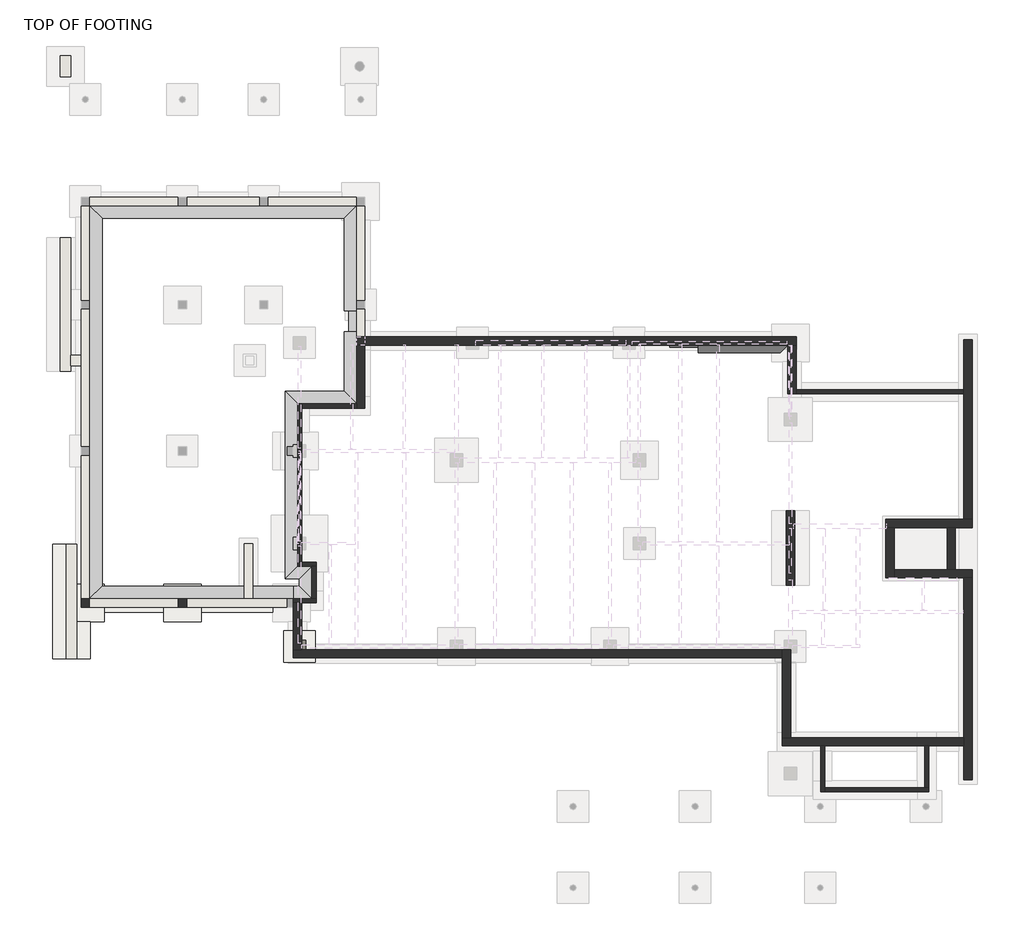
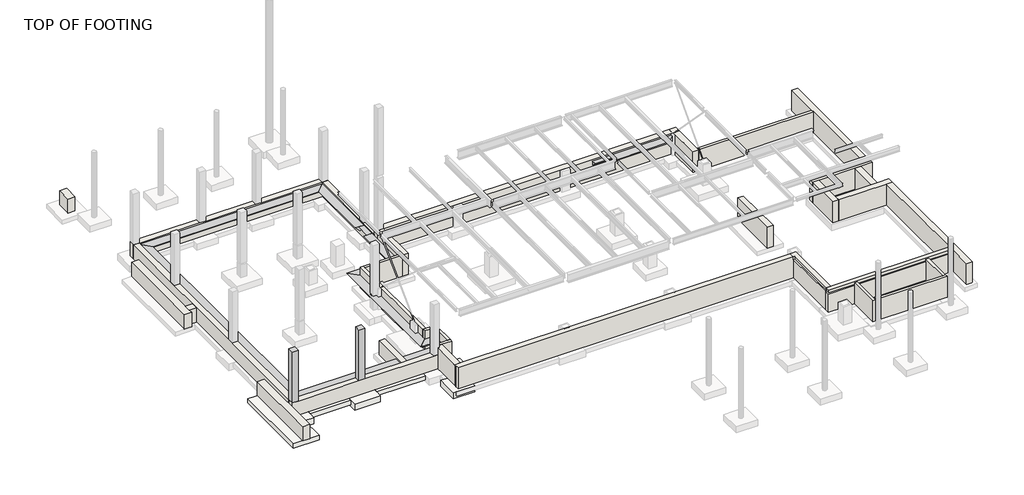
# One storey, part 1 of 4: 32 walls, 8 proxies, 3 slabs, 2 columns, 2 footings.
# Revit data of these elements (continued)
# Element 20 (IfcWall, "Foundation - 16\" Concrete") (continued)
#   RM User Number = 221
#   RM Unique Id = 1041
#   RS Unique Id = 299748
#   Phase Created = New Construction
#   Base Constraint = TOP OF FOOTING
#   Top Constraint = Ground Floor
#   Materials on its faces: "Concrete, Normal Weight - 4 ksi"
# Element 21 (IfcWall, "Foundation - 16\" Concrete")
#   Comments = ""
#   Top Offset = 0 mm
#   Base Offset = 0 mm
#   wall height = 1574.8 mm
#   RM User Number = 222
#   RM Unique Id = 1042
#   RS Unique Id = 299919
#   Phase Created = New Construction
#   Base Constraint = TOP OF FOOTING
#   Top Constraint = Ground Floor
#   Materials on its faces: "Concrete, Normal Weight - 4 ksi"
# Element 22 (IfcWall, "Foundation - 16\" Concrete")
#   Comments = ""
#   Top Offset = 0 mm
#   Base Offset = 0 mm
#   wall height = 1066.8 mm
#   RM User Number = 223
#   RM Unique Id = 1043
#   RS Unique Id = 300105
#   Phase Created = New Construction
#   Base Constraint = TOP OF FOOTING
#   Top Constraint = LOWER LEVEL
#   Materials on its faces: "Concrete, Normal Weight - 4 ksi"
# Element 23 (IfcWall, "Foundation - 16\" Concrete")
#   Comments = ""
#   Top Offset = 0 mm
#   Base Offset = 0 mm
#   wall height = 1066.8 mm
#   RM User Number = 224
#   RM Unique Id = 1044
#   RS Unique Id = 300160
#   Phase Created = New Construction
#   Base Constraint = TOP OF FOOTING
#   Top Constraint = LOWER LEVEL
#   Materials on its faces: "Concrete, Normal Weight - 4 ksi"
# Element 24 (IfcWall, "Foundation - 16\" Concrete")
#   Comments = ""
#   Top Offset = 0 mm
#   Base Offset = 0 mm
#   wall height = 1066.8 mm
#   RM User Number = 225
#   RM Unique Id = 1045
#   RS Unique Id = 300261
#   Phase Created = New Construction
#   Base Constraint = TOP OF FOOTING
#   Top Constraint = LOWER LEVEL
#   Materials on its faces: "Concrete, Normal Weight - 4 ksi"
# Element 25 (IfcWall, "Foundation - 16\" Concrete")
#   Comments = ""
#   Top Offset = 0 mm
#   Base Offset = 0 mm
#   wall height = 1066.8 mm
#   RM User Number = 226
#   RM Unique Id = 1046
#   RS Unique Id = 300335
#   Phase Created = New Construction
#   Base Constraint = TOP OF FOOTING
#   Top Constraint = LOWER LEVEL
#   Materials on its faces: "Concrete, Normal Weight - 4 ksi"
# Element 26 (IfcWall, "Foundation - 16\" Concrete")
#   Comments = ""
#   Top Offset = 0 mm
#   Base Offset = 0 mm
#   wall height = 1574.8 mm
#   RM User Number = 228
#   RM Unique Id = 1048
#   RS Unique Id = 300755
#   Phase Created = New Construction
#   Base Constraint = TOP OF FOOTING
#   Top Constraint = Ground Floor
#   Materials on its faces: "Concrete, Normal Weight - 4 ksi", "Concrete, Cast-in-Place gray"
# Element 27 (IfcWall, "Foundation - 16\" Concrete")
#   Comments = ""
#   Top Offset = 0 mm
#   Base Offset = 0 mm
#   wall height = 1574.8 mm
#   RM User Number = 231
#   RM Unique Id = 1055
#   RS Unique Id = 301226
#   Phase Created = New Construction
#   Base Constraint = TOP OF FOOTING
#   Top Constraint = Ground Floor
#   Materials on its faces: "Concrete, Normal Weight - 4 ksi"
# Element 28 (IfcWall, "Foundation - 16\" Concrete")
#   Comments = ""
#   Top Offset = 0 mm
#   Base Offset = 0 mm
#   wall height = 1574.8 mm
#   RM User Number = 232
#   RM Unique Id = 1056
#   RS Unique Id = 301303
#   Phase Created = New Construction
#   Base Constraint = TOP OF FOOTING
#   Top Constraint = Ground Floor
#   Materials on its faces: "Concrete, Normal Weight - 4 ksi"
# Element 29 (IfcWall, "Foundation - 16\" Concrete")
#   Comments = ""
#   Top Offset = 0 mm
#   Base Offset = 0 mm
#   wall height = 1574.8 mm
#   RM User Number = 233
#   RM Unique Id = 1057
#   RS Unique Id = 301434
#   Phase Created = New Construction
#   Base Constraint = TOP OF FOOTING
#   Top Constraint = Ground Floor
#   Materials on its faces: "Concrete, Normal Weight - 4 ksi"
# Element 30 (IfcWall, "Foundation - 16\" Concrete")
#   Comments = ""
#   Top Offset = 0 mm
#   Base Offset = 0 mm
#   wall height = 1066.8 mm
#   RM User Number = 252
#   RM Unique Id = 1092
#   RS Unique Id = 386049
#   Phase Created = New Construction
#   Base Constraint = TOP OF FOOTING
#   Top Constraint = LOWER LEVEL
#   Materials on its faces: "Concrete, Normal Weight - 4 ksi"
# Element 31 (IfcWall, "Foundation - 16\" Concrete")
#   Top Offset = 0 mm
#   Base Offset = 0 mm
#   wall height = 1574.8 mm
#   RM User Number = 253
#   RM Unique Id = 1093
#   RS Unique Id = 386870
#   Phase Created = New Construction
#   Base Constraint = TOP OF FOOTING
#   Top Constraint = Ground Floor
#   Materials on its faces: "Concrete, Normal Weight - 4 ksi"
# Element 32 (IfcWall, "Foundation - 16\" Concrete")
#   Comments = ""
#   Top Offset = 0 mm
#   Base Offset = 0 mm
#   wall height = 1574.8 mm
#   RM User Number = 261
#   RM Unique Id = 1108
#   RS Unique Id = 398252
#   Phase Created = New Construction
#   Base Constraint = TOP OF FOOTING
#   Top Constraint = Ground Floor
#   Materials on its faces: "Concrete, Normal Weight - 4 ksi"
# Element 33 (IfcWall, "Foundation - 16\" Concrete w/Brick Ledge")
#   Comments = ""
#   Top Offset = 0 mm
#   Base Offset = 0 mm
#   wall height = 1574.8 mm
#   RM User Number = 218
#   RM Unique Id = 1036
#   RS Unique Id = 299490
#   Phase Created = New Construction
#   Base Constraint = TOP OF FOOTING
#   Top Constraint = Ground Floor
#   Materials on its faces: "Concrete, Cast-in-Place gray"
# Element 34 (IfcWall, "Foundation - 16\" Concrete w/Brick Ledge")
#   Comments = ""
#   Top Offset = 0 mm
#   Base Offset = 0 mm
#   wall height = 1574.8 mm
#   RM User Number = 219
#   RM Unique Id = 1039
#   RS Unique Id = 299551
#   Phase Created = New Construction
#   Base Constraint = TOP OF FOOTING
#   Top Constraint = Ground Floor
#   Materials on its faces: "Concrete, Cast-in-Place gray", "Concrete, Normal Weight - 4 ksi"
# Element 35 (IfcWall, "Foundation - 20\" Concrete")
#   Comments = ""
#   Top Offset = 0 mm
#   Base Offset = 0 mm
#   wall height = 1066.8 mm
#   RM User Number = 249
#   RM Unique Id = 1087
#   RS Unique Id = 384622
#   Phase Created = New Construction
#   Base Constraint = TOP OF FOOTING
#   Top Constraint = LOWER LEVEL
#   Materials on its faces: "Concrete, Cast-in-Place gray"
# Element 36 (IfcWall, "Foundation - 20\" Concrete")
#   Top Offset = 0 mm
#   Base Offset = 0 mm
#   wall height = 1066.8 mm
#   RM User Number = 250
#   RM Unique Id = 1090
#   RS Unique Id = 385305
#   Phase Created = New Construction
#   Base Constraint = TOP OF FOOTING
#   Top Constraint = LOWER LEVEL
#   Materials on its faces: "Concrete, Cast-in-Place gray"
# Element 37 (IfcWall, "Foundation - 20\" Concrete")
#   Comments = ""
#   Top Offset = 0 mm
#   Base Offset = 0 mm
#   wall height = 1066.8 mm
#   RM User Number = 251
#   RM Unique Id = 1091
#   RS Unique Id = 385646
#   Phase Created = New Construction
#   Base Constraint = TOP OF FOOTING
#   Top Constraint = LOWER LEVEL
#   Materials on its faces: "Concrete, Cast-in-Place gray"
# Element 38 (IfcWall, "Foundation - 20\" Concrete")
#   Top Offset = 0 mm
#   Base Offset = 0 mm
#   wall height = 1066.8 mm
#   Phase Created = New Construction
#   Base Constraint = TOP OF FOOTING
#   Top Constraint = LOWER LEVEL
#   Materials on its faces: "Concrete, Cast-in-Place gray"
# Element 39 (IfcWall, "Foundation - 8\" Concrete")
#   Comments = ""
#   Top Offset = 0 mm
#   Base Offset = 0 mm
#   wall height = 1574.8 mm
#   RM User Number = 216
#   RM Unique Id = 1032
#   RS Unique Id = 299171
#   Phase Created = New Construction
#   Base Constraint = TOP OF FOOTING
#   Top Constraint = Ground Floor
#   Materials on its faces: "Concrete, Cast-in-Place gray"
# Element 40 (IfcWall, "Foundation - 8\" Concrete")
#   Comments = ""
#   Top Offset = 0 mm
#   Base Offset = 0 mm
#   wall height = 1574.8 mm
#   RM User Number = 227
#   RM Unique Id = 1047
#   RS Unique Id = 300517
#   Phase Created = New Construction
#   Base Constraint = TOP OF FOOTING
#   Top Constraint = Ground Floor
#   Materials on its faces: "Concrete, Cast-in-Place gray"
# Element 41 (IfcWall, "Foundation - 8\" Concrete")
#   Comments = ""
#   Mark = ""
#   Top Offset = 0 mm
#   Base Offset = 0 mm
#   wall height = 1574.8 mm
#   RM User Number = 229
#   RM Unique Id = 1049
#   RS Unique Id = 300795
#   Phase Created = New Construction
#   Base Constraint = TOP OF FOOTING
#   Top Constraint = Ground Floor
#   Materials on its faces: "Concrete, Cast-in-Place gray"
# Element 42 (IfcWall, "Foundation - 8\" Concrete")
#   Top Offset = 0 mm
#   Base Offset = 0 mm
#   wall height = 1574.8 mm
#   RM User Number = 238
#   RM Unique Id = 1072
#   RS Unique Id = 306635
#   Phase Created = New Construction
#   Base Constraint = TOP OF FOOTING
#   Top Constraint = Ground Floor
#   Materials on its faces: "Concrete, Cast-in-Place gray"
# Element 43 (IfcWall, "Foundation - 8\" Concrete")
#   Top Offset = 0 mm
#   Base Offset = 0 mm
#   wall height = 1574.8 mm
#   RM User Number = 239
#   RM Unique Id = 1073
#   RS Unique Id = 306730
#   Phase Created = New Construction
#   Base Constraint = TOP OF FOOTING
#   Top Constraint = Ground Floor
#   Materials on its faces: "Concrete, Cast-in-Place gray"
# Element 44 (IfcWall, "Foundation - 8\" Concrete")
#   Top Offset = 0 mm
#   Base Offset = 0 mm
#   wall height = 1574.8 mm
#   RM User Number = 240
#   RM Unique Id = 1074
#   RS Unique Id = 306817
#   Phase Created = New Construction
#   Base Constraint = TOP OF FOOTING
#   Top Constraint = Ground Floor
#   Materials on its faces: "Concrete, Cast-in-Place gray", "Concrete, Normal Weight - 4 ksi"
# Element 45 (IfcWall, "Foundation - 8\" Concrete")
#   Comments = ""
#   Top Offset = 0 mm
#   Base Offset = 0 mm
#   wall height = 1574.8 mm
#   RM User Number = 241
#   RM Unique Id = 1075
#   RS Unique Id = 308422
#   Phase Created = New Construction
#   Base Constraint = TOP OF FOOTING
#   Top Constraint = Ground Floor
#   Materials on its faces: "Concrete, Cast-in-Place gray"
# Element 46 (IfcWall, "Foundation - 8\" Concrete")
#   Comments = ""
#   Top Offset = 0 mm
#   Base Offset = 0 mm
#   wall height = 1574.8 mm
#   RM User Number = 242
#   RM Unique Id = 1076
#   RS Unique Id = 308469
#   Phase Created = New Construction
#   Base Constraint = TOP OF FOOTING
#   Top Constraint = Ground Floor
#   Materials on its faces: "Concrete, Cast-in-Place gray"
# Element 47 (IfcWall, "Foundation - 8\" Concrete")
#   Comments = ""
#   Top Offset = 0 mm
#   Base Offset = 0 mm
#   wall height = 1574.8 mm
#   RM User Number = 243
#   RM Unique Id = 1077
#   RS Unique Id = 308516
#   Phase Created = New Construction
#   Base Constraint = TOP OF FOOTING
#   Top Constraint = Ground Floor
#   Materials on its faces: "Concrete, Cast-in-Place gray"
# Materials
#   "Concrete, Cast-in-Place gray": class "Concrete", colour RGB 192 192 192, transparency 0, Description = "Cast-in-place concrete", Cost = 0
#   "Concrete - Cast-in-Place Concrete": class "Concrete", colour RGB 192 192 192, transparency 0
#   "Concrete, Normal Weight - 4 ksi": class "Concrete", colour RGB 192 192 192, transparency 0, Description = "Concrete 4 ksi", Cost = 0
#   "Brass, Soft Yellow, Welded": class "Metal", colour RGB 120 120 120, transparency 0, Description = "Soft yellow brass, welded", Cost = 0
